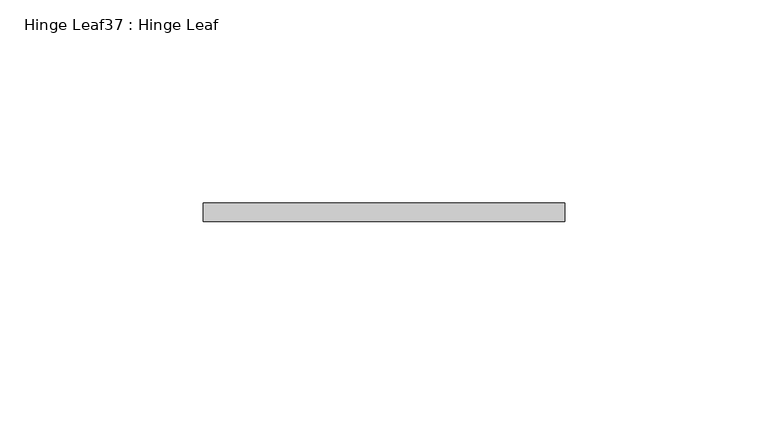
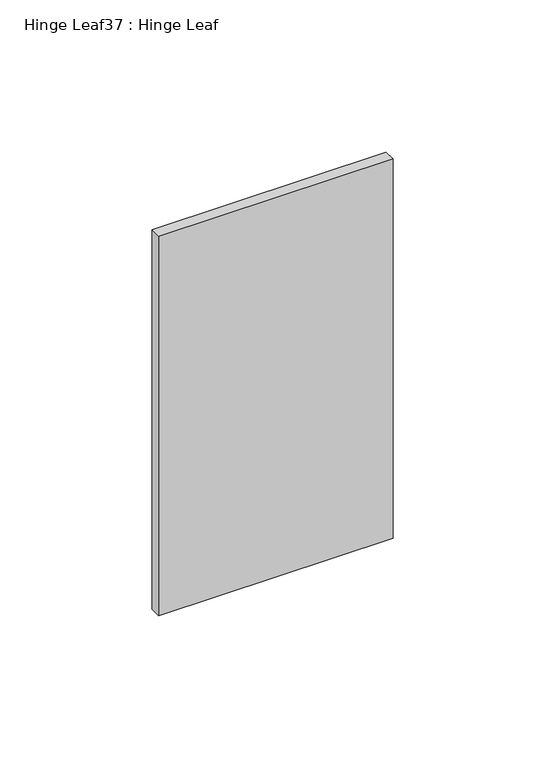
"""IFC4 building model written with IfcOpenShell, lengths in millimetres: proxy geometry, Hinge Leaf37 : Hinge Leaf."""

from ifc_helpers import new_model, si_unit, frame, origin, place, context, project, spatial, polyline, outline, extrude, source, transform, mapped, element, save


def hinge_leaf37_hinge_leaf_bf372cbc(model_context):
    return source(origin(), model_context, "Body", "SweptSolid", [
        extrude(outline(polyline([(587327.7934739, -533988.7163841), (587327.7934739, -533984.1443841), (587416.6934739, -533984.1443841), (587416.6934739, -533988.7163841), (587327.7934739, -533988.7163841)])), frame((0.0, 0.0, 1123.95), z_axis=(0.0, 0.0, 1.0), x_axis=(1.0, 0.0, 0.0)), (0.0, 0.0, 1.0), 152.4),
    ])


if __name__ == "__main__":
    model = new_model("IFC4")
    model_context = context("Model", 3, world=origin())
    ifc_project = project(units=[si_unit("LENGTHUNIT", "METRE", prefix="MILLI")], contexts=[model_context])
    site = spatial("IfcSite", under=ifc_project)
    building = spatial("IfcBuilding", under=site)
    placement = place(None, origin())
    hinge_leaf37_hinge_leaf_shape = hinge_leaf37_hinge_leaf_bf372cbc(model_context)
    element("IfcBuildingElementProxy", 1, Name="Hinge Leaf37 : Hinge Leaf", ObjectType="Hinge Leaf37 : Hinge Leaf", at=placement, inside=building, context=model_context, shape_type="MappedRepresentation", body=[
        mapped(hinge_leaf37_hinge_leaf_shape, transform((0.0, 0.0, 0.0), x_axis=(1.0, 0.0, 0.0), y_axis=(0.0, 1.0, 0.0), z_axis=(0.0, 0.0, 1.0))),
    ])
    save(model, "model.ifc")

# Revit data of these elements
# Element 1 (IfcBuildingElementProxy, "Hinge Leaf37 : Hinge Leaf")
#   Materials on its faces: "6\"X6\" WELD-ON STL BUTT HINGE"
# Materials
#   "6\"X6\" WELD-ON STL BUTT HINGE": class "Metal", colour RGB 189 187 185, transparency 0, Description = "Carbon steel", Cost = 0
